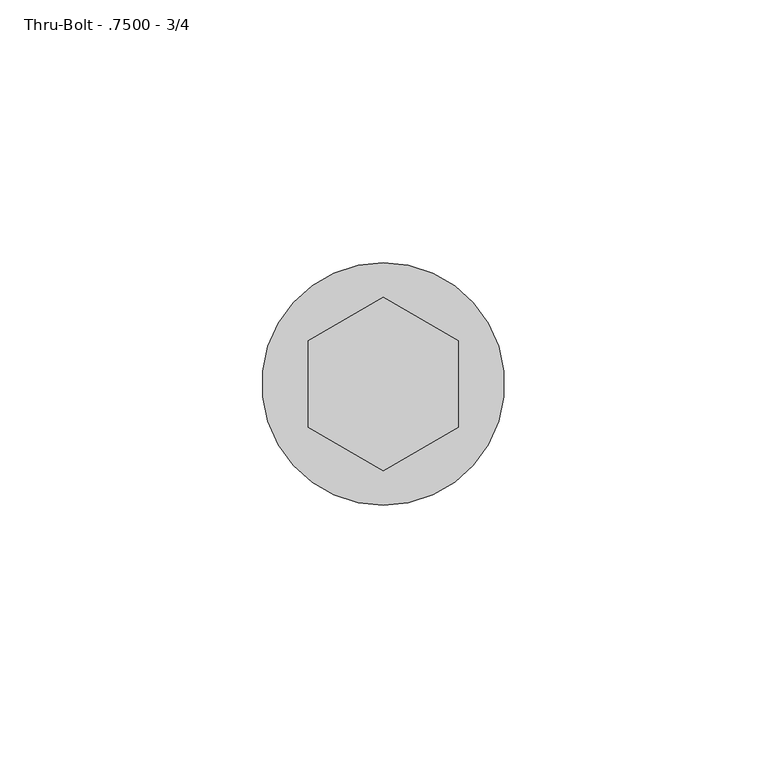
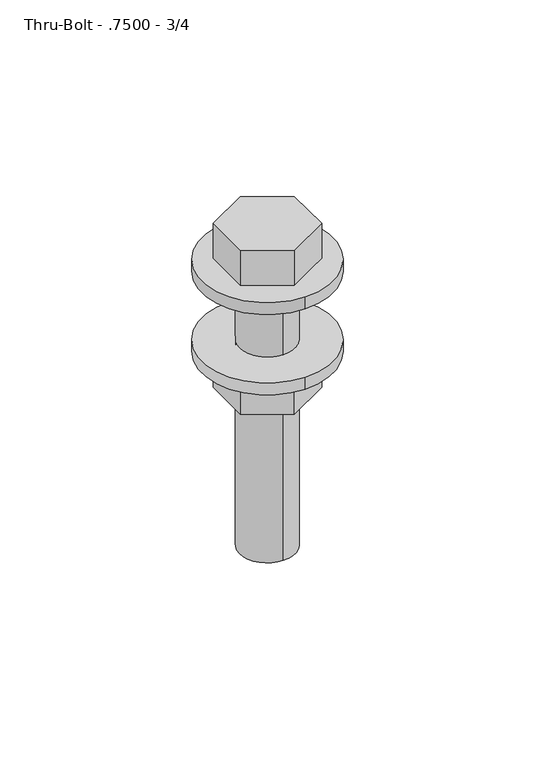
"""IFC4 building model written with IfcOpenShell, lengths in millimetres: fastener geometry, 060523 - W_P_C - Fastenings - Generic : Thru-Bolt - .7500 - 3/4."""

from ifc_helpers import new_model, si_unit, point, frame, origin, origin_with_axes, origin_2d, place, context, project, spatial, polyline, circle_curve, trimmed, segment, composite_curve, outline, extrude, source, transform, mapped, element, save


def thru_bolt_7500_3_4_4b407497(model_context):
    return source(origin(), model_context, "Body", "SweptSolid", [
        extrude(outline(composite_curve([segment(trimmed(circle_curve(origin_2d(), 23.0683594), [point((0.0, 23.0683594))], [point((0.0, -23.0683594))], False, "CARTESIAN"), True, "CONTINUOUS"), segment(trimmed(circle_curve(origin_2d(), 23.0683594), [point((0.0, -23.0683594))], [point((0.0, 23.0683594))], False, "CARTESIAN"), True, "CONTINUOUS")], self_intersect=False)), origin_with_axes(), (0.0, 0.0, 1.0), 4.4317708),
        extrude(outline(composite_curve([segment(trimmed(circle_curve(origin_2d(), 23.0683594), [point((0.0, 23.0683594))], [point((0.0, -23.0683594))], False, "CARTESIAN"), True, "CONTINUOUS"), segment(trimmed(circle_curve(origin_2d(), 23.0683594), [point((0.0, -23.0683594))], [point((0.0, 23.0683594))], False, "CARTESIAN"), True, "CONTINUOUS")], self_intersect=False)), frame((0.0, 0.0, -29.8317708), z_axis=(0.0, 0.0, 1.0), x_axis=(1.0, 0.0, 0.0)), (0.0, 0.0, 1.0), 4.4317708),
        extrude(outline(polyline([(-14.2875, -8.248892), (-14.2875, 8.248892), (0.0, 16.4977839), (14.2875, 8.248892), (14.2875, -8.248892), (0.0, -16.4977839), (-14.2875, -8.248892)])), frame((0.0, 0.0, -43.1270833), z_axis=(0.0, 0.0, 1.0), x_axis=(1.0, 0.0, 0.0)), (0.0, 0.0, 1.0), 13.2953125),
        extrude(outline(polyline([(-14.2875, 8.248892), (0.0, 16.4977839), (14.2875, 8.248892), (14.2875, -8.248892), (0.0, -16.4977839), (-14.2875, -8.248892), (-14.2875, 8.248892)])), frame((0.0, 0.0, 4.4317708), z_axis=(0.0, 0.0, 1.0), x_axis=(1.0, 0.0, 0.0)), (0.0, 0.0, 1.0), 13.2953125),
        extrude(outline(composite_curve([segment(trimmed(circle_curve(origin_2d(), 9.7730469), [point((0.0, -9.7730469))], [point((0.0, 9.7730469))], False, "CARTESIAN"), True, "CONTINUOUS"), segment(trimmed(circle_curve(origin_2d(), 9.7730469), [point((0.0, 9.7730469))], [point((0.0, -9.7730469))], False, "CARTESIAN"), True, "CONTINUOUS")], self_intersect=False)), frame((0.0, 0.0, -101.6), z_axis=(0.0, 0.0, 1.0), x_axis=(1.0, 0.0, 0.0)), (0.0, 0.0, 1.0), 106.0317708),
    ])


if __name__ == "__main__":
    model = new_model("IFC4")
    model_context = context("Model", 3, world=origin())
    ifc_project = project(units=[si_unit("LENGTHUNIT", "METRE", prefix="MILLI")], contexts=[model_context])
    site = spatial("IfcSite", under=ifc_project)
    building = spatial("IfcBuilding", under=site)
    placement = place(None, origin())
    thru_bolt_7500_3_4_shape = thru_bolt_7500_3_4_4b407497(model_context)
    element("IfcFastener", 1, ObjectType="060523 - W_P_C - Fastenings - Generic : Thru-Bolt - .7500 - 3/4", at=placement, inside=building, context=model_context, shape_type="MappedRepresentation", body=[
        mapped(thru_bolt_7500_3_4_shape, transform((0.0, 0.0, 0.0), x_axis=(1.0, 0.0, 0.0), y_axis=(0.0, 1.0, 0.0), z_axis=(0.0, 0.0, 1.0))),
    ])
    save(model, "model.ifc")

# Revit data of these elements
# Type "060523 - W_P_C - Fastenings - Generic : Thru-Bolt - .7500 - 3/4"
#   Washer_Thickness = 0' - 0.17448"
#   Washer Radius = 0' - 0.9082"
#   Washer Offset - Head = 0' - 0.17448"
#   Washer Offset = 0' - 0.17448"
#   Thickness_of_Substrate [instance default] = 0' - 1"
#   Side = 0' - 0.65039"
#   Radius = 0' - 0.38477"
#   Length [instance default] = 0' - 4"
#   Head Size = 0' - 1 1/8"
#   Head Radius = 0' - 0 9/16"
#   Head Height = 0' - 0 67/128"
#   Double Diameter = 0' - 1 69/128"
#   Diameter = 0' - 0 197/256"
#   Default Elevation = 4' - 0"
#   Washer_Nut_Visibility = yes
#   Washer_Head_Visibility = yes
#   Round_Head_Visibility = no
#   Point Visibility = no
#   Nut_Visibility = yes
#   Hex_Head_Visiblilty = yes
#   Washer Material = none
#   Bolt Material (Size) = AT SILL - FASTENER AT 24" O.C.
# Element 1 (IfcFastener, "060523 - W_P_C - Fastenings - Generic : Thru-Bolt - .7500 - 3/4")
#   Materials on its faces: "AT SILL - FASTENER AT 24\" O.C."
# Materials
#   "AT SILL - FASTENER AT 24\" O.C.": class "Generic", colour RGB 120 120 120, transparency 0, Cost = 0
